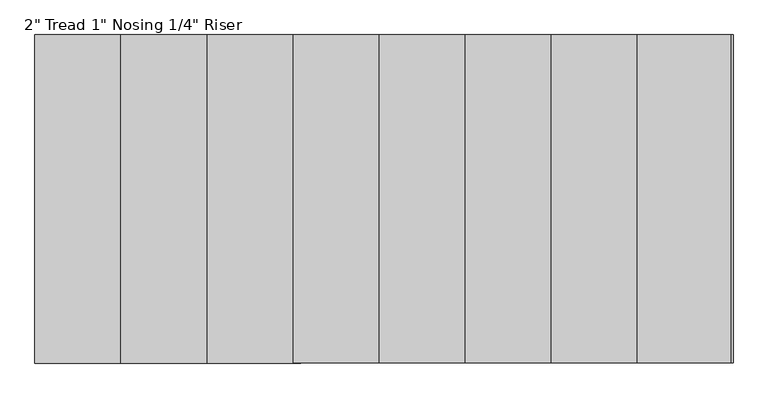
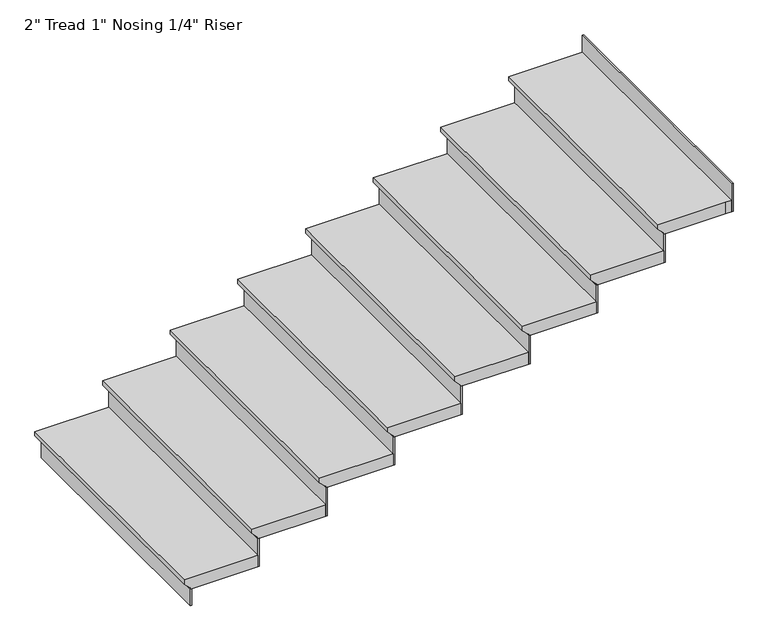
"""IFC4 building model written with IfcOpenShell, lengths in millimetres: stair flight geometry."""

from ifc_helpers import new_model, si_unit, origin, place, context, project, spatial, faceted_brep, source, transform, mapped, element, save


def stair_flight_46f433d9(model_context):
    return source(origin(), model_context, "Body", "Brep", [
        faceted_brep([(663721.188677, -551651.2413841, 104.5175676), (663721.188677, -551651.2413841, 123.5675676), (663721.188677, -550584.4413841, 123.5675676), (663721.188677, -550584.4413841, 104.5175676), (663746.588677, -551651.2413841, 79.1175676), (663746.588677, -550584.4413841, 79.1175676), (664025.988677, -551651.2413841, 123.5675676), (664025.988677, -550584.4413841, 123.5675676), (663746.588677, -550584.4413841, 72.7675676), (664025.988677, -550584.4413841, 72.7675676), (664025.988677, -551651.2413841, 72.7675676), (663746.588677, -551651.2413841, 72.7675676)], [[[0, 1, 2, 3]], [[4, 0, 3, 5]], [[2, 1, 6, 7]], [[8, 9, 10, 11]], [[2, 7, 9, 8, 5, 3]], [[8, 11, 4, 5]], [[6, 1, 0, 4, 11, 10]], [[7, 6, 10, 9]]]),
        faceted_brep([(663746.588677, -551651.2413841, 72.7675676), (663746.588677, -551651.2413841, 0.0), (663752.938677, -551651.2413841, 0.0), (663752.938677, -551651.2413841, 72.7675676), (663746.588677, -550584.4413841, 72.7675676), (663752.938677, -550584.4413841, 72.7675676), (663752.938677, -550584.4413841, 0.0), (663746.588677, -550584.4413841, 0.0)], [[[0, 1, 2, 3]], [[4, 5, 6, 7]], [[1, 0, 4, 7]], [[2, 1, 7, 6]], [[3, 2, 6, 5]], [[0, 3, 5, 4]]]),
        faceted_brep([(664025.988677, -551651.2413841, 196.3351351), (664025.988677, -551651.2413841, 72.7675676), (664032.338677, -551651.2413841, 72.7675676), (664032.338677, -551651.2413841, 196.3351351), (664025.988677, -550584.4413841, 196.3351351), (664032.338677, -550584.4413841, 196.3351351), (664032.338677, -550584.4413841, 72.7675676), (664025.988677, -550584.4413841, 72.7675676)], [[[0, 1, 2, 3]], [[4, 5, 6, 7]], [[1, 0, 4, 7]], [[2, 1, 7, 6]], [[3, 2, 6, 5]], [[0, 3, 5, 4]]]),
        faceted_brep([(664000.588677, -550584.4413841, 247.1351351), (664000.588677, -551651.2413841, 247.1351351), (664305.388677, -551651.2413841, 247.1351351), (664305.388677, -550584.4413841, 247.1351351), (664025.988677, -550584.4413841, 196.3351351), (664305.388677, -550584.4413841, 196.3351351), (664305.388677, -551651.2413841, 196.3351351), (664025.988677, -551651.2413841, 196.3351351), (664025.988677, -550584.4413841, 202.6851351), (664000.588677, -550584.4413841, 228.0851351), (664025.988677, -551651.2413841, 202.6851351), (664000.588677, -551651.2413841, 228.0851351)], [[[0, 1, 2, 3]], [[4, 5, 6, 7]], [[0, 3, 5, 4, 8, 9]], [[4, 7, 10, 8]], [[2, 1, 11, 10, 7, 6]], [[3, 2, 6, 5]], [[11, 1, 0, 9]], [[10, 11, 9, 8]]]),
        faceted_brep([(664305.388677, -551651.2413841, 319.9027027), (664305.388677, -551651.2413841, 196.3351351), (664311.738677, -551651.2413841, 196.3351351), (664311.738677, -551651.2413841, 319.9027027), (664305.388677, -550584.4413841, 319.9027027), (664311.738677, -550584.4413841, 319.9027027), (664311.738677, -550584.4413841, 196.3351351), (664305.388677, -550584.4413841, 196.3351351)], [[[0, 1, 2, 3]], [[4, 5, 6, 7]], [[1, 0, 4, 7]], [[2, 1, 7, 6]], [[3, 2, 6, 5]], [[0, 3, 5, 4]]]),
        faceted_brep([(664279.988677, -550584.4413841, 370.7027027), (664279.988677, -551651.2413841, 370.7027027), (664584.788677, -551651.2413841, 370.7027027), (664584.788677, -550584.4413841, 370.7027027), (664305.388677, -550584.4413841, 319.9027027), (664584.788677, -550584.4413841, 319.9027027), (664584.788677, -551651.2413841, 319.9027027), (664305.388677, -551651.2413841, 319.9027027), (664305.388677, -550584.4413841, 326.2527027), (664279.988677, -550584.4413841, 351.6527027), (664305.388677, -551651.2413841, 326.2527027), (664279.988677, -551651.2413841, 351.6527027)], [[[0, 1, 2, 3]], [[4, 5, 6, 7]], [[0, 3, 5, 4, 8, 9]], [[4, 7, 10, 8]], [[2, 1, 11, 10, 7, 6]], [[3, 2, 6, 5]], [[11, 1, 0, 9]], [[10, 11, 9, 8]]]),
        faceted_brep([(664584.788677, -551651.2413841, 443.4702703), (664584.788677, -551651.2413841, 319.9027027), (664591.138677, -551651.2413841, 319.9027027), (664591.138677, -551651.2413841, 443.4702703), (664584.788677, -550584.4413841, 443.4702703), (664591.138677, -550584.4413841, 443.4702703), (664591.138677, -550584.4413841, 319.9027027), (664584.788677, -550584.4413841, 319.9027027)], [[[0, 1, 2, 3]], [[4, 5, 6, 7]], [[1, 0, 4, 7]], [[2, 1, 7, 6]], [[3, 2, 6, 5]], [[0, 3, 5, 4]]]),
        faceted_brep([(664559.388677, -550584.4413841, 494.2702703), (664559.388677, -551651.2413841, 494.2702703), (664864.188677, -551651.2413841, 494.2702703), (664864.188677, -550584.4413841, 494.2702703), (664584.788677, -550584.4413841, 443.4702703), (664864.188677, -550584.4413841, 443.4702703), (664864.188677, -551651.2413841, 443.4702703), (664584.788677, -551651.2413841, 443.4702703), (664584.788677, -550584.4413841, 449.8202703), (664559.388677, -550584.4413841, 475.2202703), (664584.788677, -551651.2413841, 449.8202703), (664559.388677, -551651.2413841, 475.2202703)], [[[0, 1, 2, 3]], [[4, 5, 6, 7]], [[0, 3, 5, 4, 8, 9]], [[4, 7, 10, 8]], [[2, 1, 11, 10, 7, 6]], [[3, 2, 6, 5]], [[11, 1, 0, 9]], [[10, 11, 9, 8]]]),
        faceted_brep([(664864.188677, -551651.2413841, 567.0378378), (664864.188677, -551651.2413841, 443.4702703), (664870.538677, -551651.2413841, 443.4702703), (664870.538677, -551651.2413841, 567.0378378), (664864.188677, -550584.4413841, 567.0378378), (664870.538677, -550584.4413841, 567.0378378), (664870.538677, -550584.4413841, 443.4702703), (664864.188677, -550584.4413841, 443.4702703)], [[[0, 1, 2, 3]], [[4, 5, 6, 7]], [[1, 0, 4, 7]], [[2, 1, 7, 6]], [[3, 2, 6, 5]], [[0, 3, 5, 4]]]),
        faceted_brep([(664838.788677, -550584.4413841, 617.8378378), (664838.788677, -551651.2413841, 617.8378378), (665143.588677, -551651.2413841, 617.8378378), (665143.588677, -550584.4413841, 617.8378378), (664864.188677, -550584.4413841, 567.0378378), (665143.588677, -550584.4413841, 567.0378378), (665143.588677, -551651.2413841, 567.0378378), (664864.188677, -551651.2413841, 567.0378378), (664864.188677, -550584.4413841, 573.3878378), (664838.788677, -550584.4413841, 598.7878378), (664864.188677, -551651.2413841, 573.3878378), (664838.788677, -551651.2413841, 598.7878378)], [[[0, 1, 2, 3]], [[4, 5, 6, 7]], [[0, 3, 5, 4, 8, 9]], [[4, 7, 10, 8]], [[2, 1, 11, 10, 7, 6]], [[3, 2, 6, 5]], [[11, 1, 0, 9]], [[10, 11, 9, 8]]]),
        faceted_brep([(665143.588677, -551651.2413841, 690.6054054), (665143.588677, -551651.2413841, 567.0378378), (665149.938677, -551651.2413841, 567.0378378), (665149.938677, -551651.2413841, 690.6054054), (665143.588677, -550584.4413841, 690.6054054), (665149.938677, -550584.4413841, 690.6054054), (665149.938677, -550584.4413841, 567.0378378), (665143.588677, -550584.4413841, 567.0378378)], [[[0, 1, 2, 3]], [[4, 5, 6, 7]], [[1, 0, 4, 7]], [[2, 1, 7, 6]], [[3, 2, 6, 5]], [[0, 3, 5, 4]]]),
        faceted_brep([(665118.188677, -550584.4413841, 741.4054054), (665118.188677, -551651.2413841, 741.4054054), (665422.988677, -551651.2413841, 741.4054054), (665422.988677, -550584.4413841, 741.4054054), (665143.588677, -550584.4413841, 690.6054054), (665422.988677, -550584.4413841, 690.6054054), (665422.988677, -551651.2413841, 690.6054054), (665143.588677, -551651.2413841, 690.6054054), (665143.588677, -550584.4413841, 696.9554054), (665118.188677, -550584.4413841, 722.3554054), (665143.588677, -551651.2413841, 696.9554054), (665118.188677, -551651.2413841, 722.3554054)], [[[0, 1, 2, 3]], [[4, 5, 6, 7]], [[0, 3, 5, 4, 8, 9]], [[4, 7, 10, 8]], [[2, 1, 11, 10, 7, 6]], [[3, 2, 6, 5]], [[11, 1, 0, 9]], [[10, 11, 9, 8]]]),
        faceted_brep([(665422.988677, -551651.2413841, 814.172973), (665422.988677, -551651.2413841, 690.6054054), (665429.338677, -551651.2413841, 690.6054054), (665429.338677, -551651.2413841, 814.172973), (665422.988677, -550584.4413841, 814.172973), (665429.338677, -550584.4413841, 814.172973), (665429.338677, -550584.4413841, 690.6054054), (665422.988677, -550584.4413841, 690.6054054)], [[[0, 1, 2, 3]], [[4, 5, 6, 7]], [[1, 0, 4, 7]], [[2, 1, 7, 6]], [[3, 2, 6, 5]], [[0, 3, 5, 4]]]),
        faceted_brep([(665397.588677, -550584.4413841, 864.972973), (665397.588677, -551651.2413841, 864.972973), (665702.388677, -551651.2413841, 864.972973), (665702.388677, -550584.4413841, 864.972973), (665422.988677, -550584.4413841, 814.172973), (665702.388677, -550584.4413841, 814.172973), (665702.388677, -551651.2413841, 814.172973), (665422.988677, -551651.2413841, 814.172973), (665422.988677, -550584.4413841, 820.522973), (665397.588677, -550584.4413841, 845.922973), (665422.988677, -551651.2413841, 820.522973), (665397.588677, -551651.2413841, 845.922973)], [[[0, 1, 2, 3]], [[4, 5, 6, 7]], [[0, 3, 5, 4, 8, 9]], [[4, 7, 10, 8]], [[2, 1, 11, 10, 7, 6]], [[3, 2, 6, 5]], [[11, 1, 0, 9]], [[10, 11, 9, 8]]]),
        faceted_brep([(665981.788677, -551651.2413841, 1061.3081081), (665981.788677, -551651.2413841, 937.7405405), (665988.138677, -551651.2413841, 937.7405405), (665988.138677, -551651.2413841, 1061.3081081), (665981.788677, -550584.4413841, 1061.3081081), (665988.138677, -550584.4413841, 1061.3081081), (665988.138677, -550584.4413841, 937.7405405), (665981.788677, -550584.4413841, 937.7405405)], [[[0, 1, 2, 3]], [[4, 5, 6, 7]], [[1, 0, 4, 7]], [[2, 1, 7, 6]], [[3, 2, 6, 5]], [[0, 3, 5, 4]]]),
        faceted_brep([(665702.388677, -551651.2413841, 937.7405405), (665702.388677, -551651.2413841, 814.172973), (665708.738677, -551651.2413841, 814.172973), (665708.738677, -551651.2413841, 937.7405405), (665702.388677, -550584.4413841, 937.7405405), (665708.738677, -550584.4413841, 937.7405405), (665708.738677, -550584.4413841, 814.172973), (665702.388677, -550584.4413841, 814.172973)], [[[0, 1, 2, 3]], [[4, 5, 6, 7]], [[1, 0, 4, 7]], [[2, 1, 7, 6]], [[3, 2, 6, 5]], [[0, 3, 5, 4]]]),
        faceted_brep([(665676.988677, -550584.4413841, 988.5405405), (665676.988677, -551651.2413841, 988.5405405), (665956.388677, -551651.2413841, 988.5405405), (665981.788677, -551651.2413841, 988.5405405), (665981.788677, -550584.4413841, 988.5405405), (665702.388677, -550584.4413841, 937.7405405), (665981.788677, -550584.4413841, 937.7405405), (665981.788677, -551651.2413841, 937.7405405), (665956.388677, -551651.2413841, 937.7405405), (665702.388677, -551651.2413841, 937.7405405), (665702.388677, -550584.4413841, 944.0905405), (665676.988677, -550584.4413841, 969.4905405), (665702.388677, -551651.2413841, 944.0905405), (665676.988677, -551651.2413841, 969.4905405)], [[[0, 1, 2, 3, 4]], [[5, 6, 7, 8, 9]], [[0, 4, 6, 5, 10, 11]], [[5, 9, 12, 10]], [[2, 1, 13, 12, 9, 8]], [[3, 2, 8, 7]], [[4, 3, 7, 6]], [[13, 1, 0, 11]], [[12, 13, 11, 10]]]),
    ])


if __name__ == "__main__":
    model = new_model("IFC4")
    model_context = context("Model", 3, world=origin())
    ifc_project = project(units=[si_unit("LENGTHUNIT", "METRE", prefix="MILLI")], contexts=[model_context])
    site = spatial("IfcSite", under=ifc_project)
    building = spatial("IfcBuilding", under=site)
    placement = place(None, origin())
    stair_flight_shape = stair_flight_46f433d9(model_context)
    element("IfcStairFlight", 1, ObjectType="2\" Tread 1\" Nosing 1/4\" Riser", at=placement, inside=building, context=model_context, shape_type="MappedRepresentation", body=[
        mapped(stair_flight_shape, transform((0.0, 0.0, 0.0), x_axis=(1.0, 0.0, 0.0), y_axis=(0.0, 1.0, 0.0), z_axis=(0.0, 0.0, 1.0))),
    ])
    save(model, "model.ifc")
